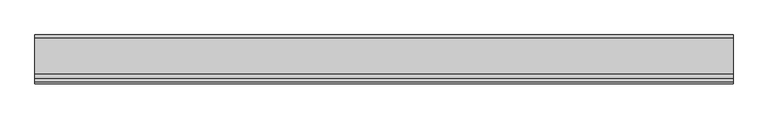
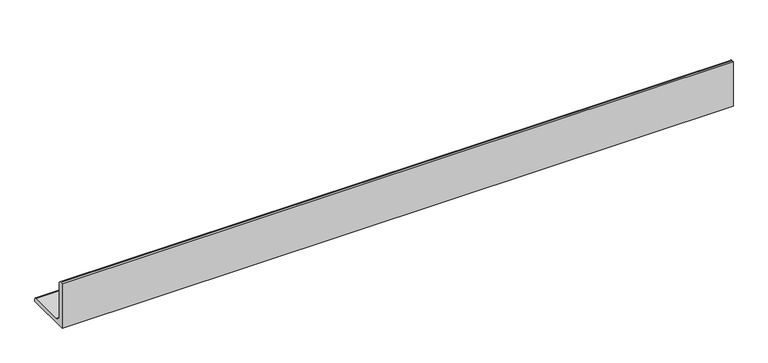
"""IFC4 building model written with IfcOpenShell, lengths in millimetres: beam geometry, NLRS_28_SF_LIB_stalen ligger hoekprofiel gelijkzijdig-AV-MMBS-SRP_gen_rsf : stalen ligger gelijkzijdig hoekprofiel LEQU_gen__150x150x15."""

from ifc_helpers import new_model, si_unit, point, frame, frame_2d, origin, place, context, project, spatial, polyline, circle_curve, trimmed, segment, composite_curve, outline, extrude, source, transform, mapped, element, save


def beam_640d1cf1(model_context):
    return source(origin(), model_context, "Body", "SweptSolid", [
        extrude(outline(composite_curve([segment(polyline([(-42.5, -42.5), (-42.5, 107.5), (-35.5, 107.5)]), True, "CONTINUOUS"), segment(trimmed(circle_curve(frame_2d((-35.5, 99.5)), 8.0), [point((-35.5, 107.5))], [point((-27.5, 99.5))], False, "CARTESIAN"), True, "CONTINUOUS"), segment(polyline([(-27.5, 99.5), (-27.5, -11.5)]), True, "CONTINUOUS"), segment(trimmed(circle_curve(frame_2d((-11.5, -11.5)), 16.0), [point((-27.5, -11.5))], [point((-11.5, -27.5))], True, "CARTESIAN"), True, "CONTINUOUS"), segment(polyline([(-11.5, -27.5), (99.5, -27.5)]), True, "CONTINUOUS"), segment(trimmed(circle_curve(frame_2d((99.5, -35.5)), 8.0), [point((99.5, -27.5))], [point((107.5, -35.5))], False, "CARTESIAN"), True, "CONTINUOUS"), segment(polyline([(107.5, -35.5), (107.5, -42.5), (-42.5, -42.5)]), True, "CONTINUOUS")], self_intersect=False)), frame((-1070.0, 0.0, 0.0), z_axis=(1.0, 0.0, 0.0), x_axis=(0.0, 1.0, 0.0)), (0.0, 0.0, 1.0), 2140.0),
    ])


if __name__ == "__main__":
    model = new_model("IFC4")
    model_context = context("Model", 3, world=origin())
    ifc_project = project(units=[si_unit("LENGTHUNIT", "METRE", prefix="MILLI")], contexts=[model_context])
    site = spatial("IfcSite", under=ifc_project)
    building = spatial("IfcBuilding", under=site)
    placement = place(None, origin())
    beam_shape = beam_640d1cf1(model_context)
    element("IfcBeam", 1, ObjectType="NLRS_28_SF_LIB_stalen ligger hoekprofiel gelijkzijdig-AV-MMBS-SRP_gen_rsf : stalen ligger gelijkzijdig hoekprofiel LEQU_gen__150x150x15", at=placement, inside=building, context=model_context, shape_type="MappedRepresentation", body=[
        mapped(beam_shape, transform((0.0, 0.0, 0.0), x_axis=(1.0, 0.0, 0.0), y_axis=(0.0, 1.0, 0.0), z_axis=(0.0, 0.0, 1.0))),
    ])
    save(model, "model.ifc")

# Revit data of these elements
# Type "NLRS_28_SF_LIB_stalen ligger hoekprofiel gelijkzijdig-AV-MMBS-SRP_gen_rsf : stalen ligger gelijkzijdig hoekprofiel LEQU_gen__150x150x15"
#   Type IfcGUID = "2CEqVLPNH8KRN7ghwV3a1U"
#   IfcExportAs = "IfcBeamType"
#   Type Comments = "L150x150x15"
#   Model = " "
#   Manufacturer = " "
#   Fire Rating = " "
#   Description = "stalen ligger L150x150x15"
#   Assembly Code = "28.11"
#   vz = 107.5 mm
#   vy = 107.5 mm
#   tw = 15 mm
#   tf = 15 mm
#   ri = 8 mm
#   ra = 16 mm
#   d = 150 mm
#   bf = 150 mm
#   NLRS_C_lengte [instance default] = 1524 mm
#   Length [instance default] = 1524 mm
#   Structural Material = NLRS_h2_staal_gen_rsf
#   Keynote = ""
# Element 1 (IfcBeam, "NLRS_28_SF_LIB_stalen ligger hoekprofiel gelijkzijdig-AV-MMBS-SRP_gen_rsf : stalen ligger gelijkzijdig hoekprofiel LEQU_gen__150x150x15")
#   NLRS_C_lengte = 2140 mm
#   Materials on its faces: "NLRS_h2_staal_gen_rsf"
# Materials
#   "NLRS_h2_staal_gen_rsf": class "H - Metaal", colour RGB 189 187 185, transparency 0, Keynote = "h2", Manufacturer = "Revit Standards Foundation", URL = "www.revitstandards.org", Description = "staal", Cost = 0
